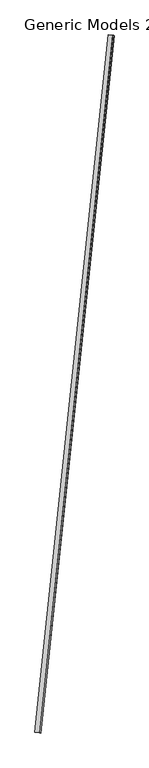
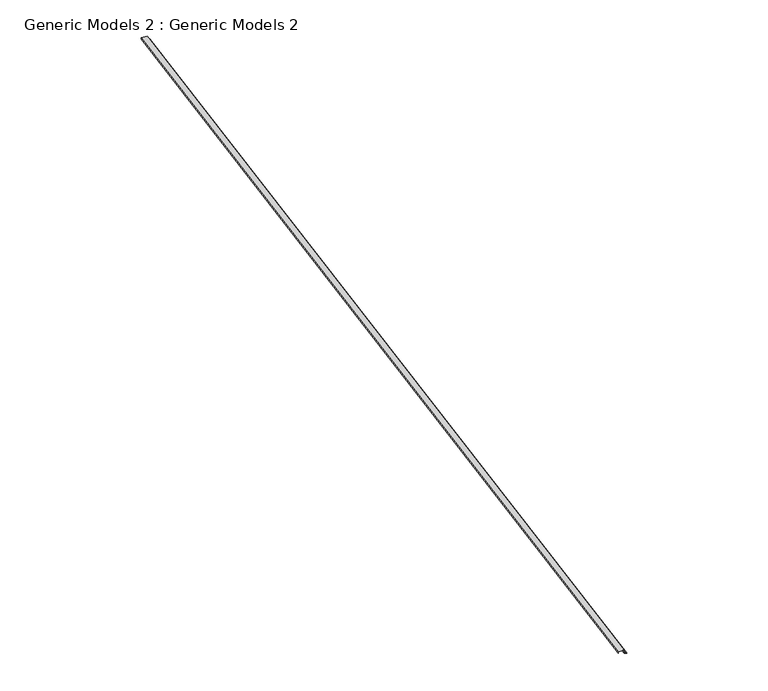
"""IFC4 building model written with IfcOpenShell, lengths in millimetres: proxy geometry, Generic Models 2 : Generic Models 2."""

from ifc_helpers import new_model, si_unit, frame, origin, place, context, project, spatial, polyline, outline, extrude, source, transform, mapped, element, save


def generic_models_2_generic_models_2_95073477(model_context):
    return source(origin(), model_context, "Body", "SweptSolid", [
        extrude(outline(polyline([(1.9726921, 0.0), (7.6651281, 1e-07), (7.6651281, -1.5874999), (1.3151281, -1.5874999), (-20.8360012, 20.5636293), (-57.3557346, -15.9561041), (-121.5366969, 48.2248582), (-103.5761847, 66.1853704), (-102.4536527, 65.0628384), (-119.2916329, 48.2248582), (-57.3557346, -13.7110401), (-20.8360012, 22.8086934), (1.9726921, 0.0)])), frame((33801.1552737, 25674.1251245, 269267.588654), z_axis=(0.10452846326765233, 0.9945218953682735, 0.0), x_axis=(0.7032331762531292, -0.073912785203537, -0.7071067811868242)), (0.0, 0.0, 1.0), 15219.520149),
    ])


if __name__ == "__main__":
    model = new_model("IFC4")
    model_context = context("Model", 3, world=origin())
    ifc_project = project(units=[si_unit("LENGTHUNIT", "METRE", prefix="MILLI")], contexts=[model_context])
    site = spatial("IfcSite", under=ifc_project)
    building = spatial("IfcBuilding", under=site)
    placement = place(None, origin())
    generic_models_2_generic_models_2_shape = generic_models_2_generic_models_2_95073477(model_context)
    element("IfcBuildingElementProxy", 1, Name="Generic Models 2 : Generic Models 2", ObjectType="Generic Models 2 : Generic Models 2", at=placement, inside=building, context=model_context, shape_type="MappedRepresentation", body=[
        mapped(generic_models_2_generic_models_2_shape, transform((0.0, 0.0, 0.0), x_axis=(1.0, 0.0, 0.0), y_axis=(0.0, 1.0, 0.0), z_axis=(0.0, 0.0, 1.0))),
    ])
    save(model, "model.ifc")

# Revit data of these elements
# Element 1 (IfcBuildingElementProxy, "Generic Models 2 : Generic Models 2")
#   Materials on its faces: "GALV. BRAKE METAL - (COLOR: DARK BRONZE)"
# Materials
#   "GALV. BRAKE METAL - (COLOR: DARK BRONZE)": class "Generic", colour RGB 72 52 47, transparency 0, Cost = 0
